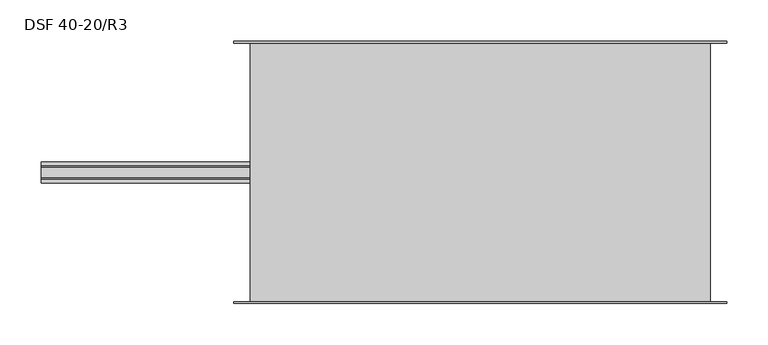
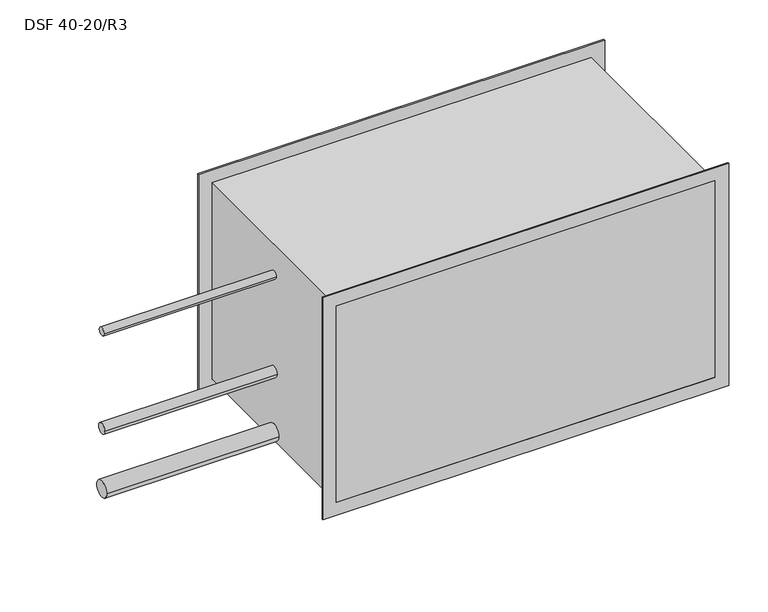
"""IFC4 building model written with IfcOpenShell, lengths in millimetres: proxy geometry, Воздухоохладитель фреоновый DSF : DSF 40-20/R3."""

from ifc_helpers import new_model, si_unit, point, frame, frame_2d, origin, place, context, project, spatial, polyline, circle_curve, trimmed, segment, composite_curve, outline, extrude, source, transform, mapped, element, save


def dsf_40_20_r3_ad9874b6(model_context):
    return source(origin(), model_context, "Body", "SweptSolid", [
        extrude(outline(composite_curve([segment(trimmed(circle_curve(frame_2d((0.0, 105.0)), 6.0), [point((-6.0, 105.0))], [point((6.0, 105.0))], False, "CARTESIAN"), True, "CONTINUOUS"), segment(trimmed(circle_curve(frame_2d((0.0, 105.0)), 6.0), [point((6.0, 105.0))], [point((-6.0, 105.0))], False, "CARTESIAN"), True, "CONTINUOUS")], self_intersect=False)), frame((-530.0, 0.0, 0.0), z_axis=(1.0, 0.0, 0.0), x_axis=(0.0, 1.0, 0.0)), (0.0, 0.0, 1.0), 252.5),
        extrude(outline(composite_curve([segment(trimmed(circle_curve(frame_2d((0.0, -139.0)), 12.5), [point((-12.5, -139.0))], [point((12.5, -139.0))], False, "CARTESIAN"), True, "CONTINUOUS"), segment(trimmed(circle_curve(frame_2d((0.0, -139.0)), 12.5), [point((12.5, -139.0))], [point((-12.5, -139.0))], False, "CARTESIAN"), True, "CONTINUOUS")], self_intersect=False)), frame((-530.0, 0.0, 0.0), z_axis=(1.0, 0.0, 0.0), x_axis=(0.0, 1.0, 0.0)), (0.0, 0.0, 1.0), 252.5),
        extrude(outline(composite_curve([segment(trimmed(circle_curve(frame_2d((0.0, -45.0)), 8.0), [point((-8.0, -45.0))], [point((8.0, -45.0))], False, "CARTESIAN"), True, "CONTINUOUS"), segment(trimmed(circle_curve(frame_2d((0.0, -45.0)), 8.0), [point((8.0, -45.0))], [point((-8.0, -45.0))], False, "CARTESIAN"), True, "CONTINUOUS")], self_intersect=False)), frame((-530.0, 0.0, 0.0), z_axis=(1.0, 0.0, 0.0), x_axis=(0.0, 1.0, 0.0)), (0.0, 0.0, 1.0), 252.5),
        extrude(outline(polyline([(172.5, 297.5), (172.5, -297.5), (-172.5, -297.5), (-172.5, 297.5), (172.5, 297.5)]), holes=[polyline([(-152.5, 277.5), (-152.5, -277.5), (152.5, -277.5), (152.5, 277.5), (-152.5, 277.5)])]), frame((0.0, 156.5, 0.0), z_axis=(0.0, 1.0, 0.0), x_axis=(0.0, 0.0, 1.0)), (0.0, 0.0, 1.0), 2.0),
        extrude(outline(polyline([(172.5, -297.5), (-172.5, -297.5), (-172.5, 297.5), (172.5, 297.5), (172.5, -297.5)]), holes=[polyline([(152.5, 277.5), (-152.5, 277.5), (-152.5, -277.5), (152.5, -277.5), (152.5, 277.5)])]), frame((0.0, -158.5, 0.0), z_axis=(0.0, 1.0, 0.0), x_axis=(0.0, 0.0, 1.0)), (0.0, 0.0, 1.0), 2.0),
        extrude(outline(polyline([(277.5, -158.5), (-277.5, -158.5), (-277.5, 158.5), (277.5, 158.5), (277.5, -158.5)])), frame((0.0, 0.0, -152.5), z_axis=(0.0, 0.0, 1.0), x_axis=(1.0, 0.0, 0.0)), (0.0, 0.0, 1.0), 305.0),
    ])


if __name__ == "__main__":
    model = new_model("IFC4")
    model_context = context("Model", 3, world=origin())
    ifc_project = project(units=[si_unit("LENGTHUNIT", "METRE", prefix="MILLI")], contexts=[model_context])
    site = spatial("IfcSite", under=ifc_project)
    building = spatial("IfcBuilding", under=site)
    placement = place(None, origin())
    dsf_40_20_r3_shape = dsf_40_20_r3_ad9874b6(model_context)
    element("IfcBuildingElementProxy", 1, Name="Воздухоохладитель фреоновый DSF : DSF 40-20/R3", ObjectType="Воздухоохладитель фреоновый DSF : DSF 40-20/R3", at=placement, inside=building, context=model_context, shape_type="MappedRepresentation", body=[
        mapped(dsf_40_20_r3_shape, transform((0.0, 0.0, 0.0), x_axis=(1.0, 0.0, 0.0), y_axis=(0.0, 1.0, 0.0), z_axis=(0.0, 0.0, 1.0))),
    ])
    save(model, "model.ifc")

# Revit data of these elements
# Type "Воздухоохладитель фреоновый DSF : DSF 40-20/R3"
#   Manufacturer = "WAER"
#   URL = "https://waer-air.com/"
#   ADSK_Наименование краткое = "DSF 40-20/R3"
#   ADSK_Наименование = "Воздухоохладитель фреоновый DSF 40-20/R3"
#   ADSK_Масса_Текст = "17.5"
#   ADSK_Марка = ""
#   ADSK_Код изделия = ""
#   ADSK_Завод-изготовитель = "WAER"
#   ADSK_Единица измерения = "шт."
#   Д = 730 mm
#   Б = 305 mm
#   А = 555 mm
#   ADSK_Размер_Ширина = 400 mm
#   ADSK_Размер_Диаметр выход = 16 mm
#   ADSK_Размер_Диаметр вход = 12 mm
#   ADSK_Размер_Диаметр_Дренаж = 25 mm
#   ADSK_Размер_Высота = 200 mm
#   ADSK_Масса = 17.5
#   ADSK_Количество = 1
#   Default Elevation = 0
#   Keynote = ""
